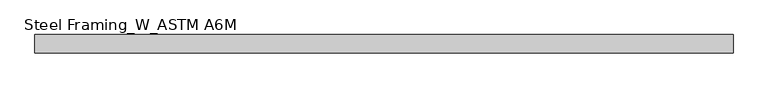
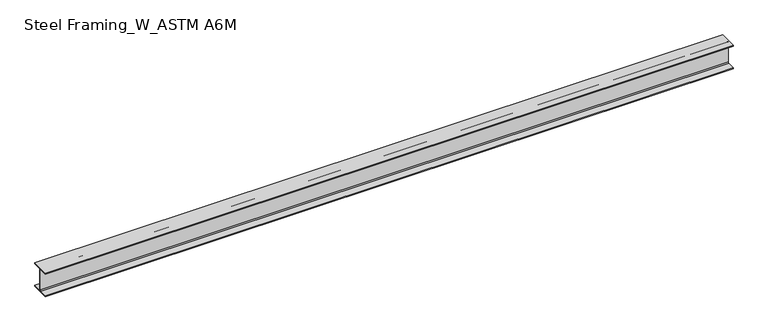
"""IFC4 building model written with IfcOpenShell, lengths in millimetres: beam geometry, Steel Framing_W_ASTM A6M : H_SB_AR_S02_W360x91_B3."""

from ifc_helpers import new_model, si_unit, point, frame, frame_2d, origin, place, context, project, spatial, polyline, circle_curve, trimmed, segment, composite_curve, outline, extrude, source, transform, mapped, element, save


def steel_framing_w_astm_a6m_17837fc5(model_context):
    return source(origin(), model_context, "Body", "SweptSolid", [
        extrude(outline(composite_curve([segment(polyline([(127.0, -160.1), (127.0, -176.5), (-127.0, -176.5), (-127.0, -160.1), (-19.865, -160.1)]), True, "CONTINUOUS"), segment(trimmed(circle_curve(frame_2d((-19.865, -145.0)), 15.1), [point((-19.865, -160.1))], [point((-4.765, -145.0))], True, "CARTESIAN"), True, "CONTINUOUS"), segment(polyline([(-4.765, -145.0), (-4.765, 145.0)]), True, "CONTINUOUS"), segment(trimmed(circle_curve(frame_2d((-19.865, 145.0)), 15.1), [point((-4.765, 145.0))], [point((-19.865, 160.1))], True, "CARTESIAN"), True, "CONTINUOUS"), segment(polyline([(-19.865, 160.1), (-127.0, 160.1), (-127.0, 176.5), (127.0, 176.5), (127.0, 160.1), (19.865, 160.1)]), True, "CONTINUOUS"), segment(trimmed(circle_curve(frame_2d((19.865, 145.0)), 15.1), [point((19.865, 160.1))], [point((4.765, 145.0))], True, "CARTESIAN"), True, "CONTINUOUS"), segment(polyline([(4.765, 145.0), (4.765, -145.0)]), True, "CONTINUOUS"), segment(trimmed(circle_curve(frame_2d((19.865, -145.0)), 15.1), [point((4.765, -145.0))], [point((19.865, -160.1))], True, "CARTESIAN"), True, "CONTINUOUS"), segment(polyline([(19.865, -160.1), (127.0, -160.1)]), True, "CONTINUOUS")], self_intersect=False)), frame((-4846.3, 0.0, 0.0), z_axis=(1.0, 0.0, 0.0), x_axis=(0.0, 1.0, 0.0)), (0.0, 0.0, 1.0), 9692.6),
    ])


if __name__ == "__main__":
    model = new_model("IFC4")
    model_context = context("Model", 3, world=origin())
    ifc_project = project(units=[si_unit("LENGTHUNIT", "METRE", prefix="MILLI")], contexts=[model_context])
    site = spatial("IfcSite", under=ifc_project)
    building = spatial("IfcBuilding", under=site)
    placement = place(None, origin())
    steel_framing_w_astm_a6m_shape = steel_framing_w_astm_a6m_17837fc5(model_context)
    element("IfcBeam", 1, ObjectType="Steel Framing_W_ASTM A6M : H_SB_AR_S02_W360x91_B3", at=placement, inside=building, context=model_context, shape_type="MappedRepresentation", body=[
        mapped(steel_framing_w_astm_a6m_shape, transform((0.0, 0.0, 0.0), x_axis=(1.0, 0.0, 0.0), y_axis=(0.0, 1.0, 0.0), z_axis=(0.0, 0.0, 1.0))),
    ])
    save(model, "model.ifc")

# Revit data of these elements
# Type "Steel Framing_W_ASTM A6M : H_SB_AR_S02_W360x91_B3"
#   Type Mark = "B3"
#   Section Name Key = "W14x61"
#   Width = 25.4 cm
#   Web Thickness = 0.953 cm
#   Web Fillet = 1.51 cm
#   Warping Constant = 1260000.0 cm⁶
#   Torsional Moment of Inertia = 91.20 cm⁴
#   Section Area = 115.0 cm²
#   Plastic Modulus weak axis = 537.0 cm³
#   Plastic Modulus strong axis = 1670.0 cm³
#   Perimeter = 1.68 m²/m
#   Nominal Weight = 91.00 kgf/m
#   Moment of Inertia weak axis = 4450.00 cm⁴
#   Moment of Inertia strong axis = 26600.00 cm⁴
#   Height = 35.3 cm
#   Flange Thickness = 1.64 cm
#   Elastic Modulus weak axis = 352.0 cm³
#   Elastic Modulus strong axis = 1510.0 cm³
#   Centroid Vertical = 17.65 cm
#   Centroid Horizontal = 12.7 cm
#   Length [instance default] = 1500 mm
#   Structural Material [instance default] = Steel, 45-345
#   Bolt Spacing = 0
#   Assembly Code = ""
# Element 1 (IfcBeam, "Steel Framing_W_ASTM A6M : H_SB_AR_S02_W360x91_B3")
#   Materials on its faces: "Steel, 45-345"
# Materials
#   "Steel, 45-345": class "Metal", colour RGB 189 187 185, transparency 0, Description = "Steel 345 MPa", Cost = 0
